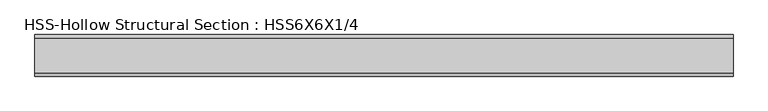
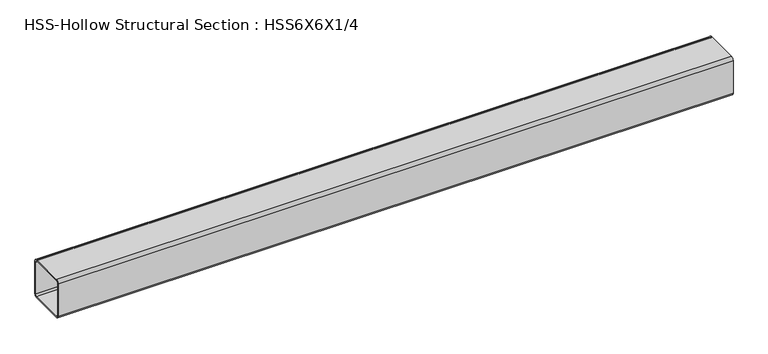
"""IFC4 building model written with IfcOpenShell, lengths in millimetres: beam geometry, HSS-Hollow Structural Section : HSS6X6X1/4."""

from ifc_helpers import new_model, si_unit, point, frame, frame_2d, origin, place, context, project, spatial, polyline, circle_curve, trimmed, segment, composite_curve, outline, extrude, source, transform, mapped, element, save


def hss_hollow_structural_section_hss6x6x1_4_a8101bfe(model_context):
    return source(origin(), model_context, "Body", "SweptSolid", [
        extrude(outline(composite_curve([segment(polyline([(76.2, 64.3636), (76.2, -64.3636)]), True, "CONTINUOUS"), segment(trimmed(circle_curve(frame_2d((64.3636, -64.3636)), 11.8364), [point((76.2, -64.3636))], [point((64.3636, -76.2))], False, "CARTESIAN"), True, "CONTINUOUS"), segment(polyline([(64.3636, -76.2), (-64.3636, -76.2)]), True, "CONTINUOUS"), segment(trimmed(circle_curve(frame_2d((-64.3636, -64.3636)), 11.8364), [point((-64.3636, -76.2))], [point((-76.2, -64.3636))], False, "CARTESIAN"), True, "CONTINUOUS"), segment(polyline([(-76.2, -64.3636), (-76.2, 64.3636)]), True, "CONTINUOUS"), segment(trimmed(circle_curve(frame_2d((-64.3636, 64.3636)), 11.8364), [point((-76.2, 64.3636))], [point((-64.3636, 76.2))], False, "CARTESIAN"), True, "CONTINUOUS"), segment(polyline([(-64.3636, 76.2), (64.3636, 76.2)]), True, "CONTINUOUS"), segment(trimmed(circle_curve(frame_2d((64.3636, 64.3636)), 11.8364), [point((64.3636, 76.2))], [point((76.2, 64.3636))], False, "CARTESIAN"), True, "CONTINUOUS")], self_intersect=False), holes=[composite_curve([segment(trimmed(circle_curve(frame_2d((-64.3636, 64.3636)), 5.9182), [point((-64.3636, 70.2818))], [point((-70.2818, 64.3636))], True, "CARTESIAN"), True, "CONTINUOUS"), segment(polyline([(-70.2818, 64.3636), (-70.2818, -64.3636)]), True, "CONTINUOUS"), segment(trimmed(circle_curve(frame_2d((-64.3636, -64.3636)), 5.9182), [point((-70.2818, -64.3636))], [point((-64.3636, -70.2818))], True, "CARTESIAN"), True, "CONTINUOUS"), segment(polyline([(-64.3636, -70.2818), (64.3636, -70.2818)]), True, "CONTINUOUS"), segment(trimmed(circle_curve(frame_2d((64.3636, -64.3636)), 5.9182), [point((64.3636, -70.2818))], [point((70.2818, -64.3636))], True, "CARTESIAN"), True, "CONTINUOUS"), segment(polyline([(70.2818, -64.3636), (70.2818, 64.3636)]), True, "CONTINUOUS"), segment(trimmed(circle_curve(frame_2d((64.3636, 64.3636)), 5.9182), [point((70.2818, 64.3636))], [point((64.3636, 70.2818))], True, "CARTESIAN"), True, "CONTINUOUS"), segment(polyline([(64.3636, 70.2818), (-64.3636, 70.2818)]), True, "CONTINUOUS")], self_intersect=False)]), frame((-1278.0540108, 0.0, 0.0), z_axis=(1.0, 0.0, 0.0), x_axis=(0.0, 1.0, 0.0)), (0.0, 0.0, 1.0), 2556.1080215),
    ])


if __name__ == "__main__":
    model = new_model("IFC4")
    model_context = context("Model", 3, world=origin())
    ifc_project = project(units=[si_unit("LENGTHUNIT", "METRE", prefix="MILLI")], contexts=[model_context])
    site = spatial("IfcSite", under=ifc_project)
    building = spatial("IfcBuilding", under=site)
    placement = place(None, origin())
    hss_hollow_structural_section_hss6x6x1_4_shape = hss_hollow_structural_section_hss6x6x1_4_a8101bfe(model_context)
    element("IfcBeam", 1, ObjectType="HSS-Hollow Structural Section : HSS6X6X1/4", at=placement, inside=building, context=model_context, shape_type="MappedRepresentation", body=[
        mapped(hss_hollow_structural_section_hss6x6x1_4_shape, transform((0.0, 0.0, 0.0), x_axis=(1.0, 0.0, 0.0), y_axis=(0.0, 1.0, 0.0), z_axis=(0.0, 0.0, 1.0))),
    ])
    save(model, "model.ifc")

# Revit data of these elements
# Type "HSS-Hollow Structural Section : HSS6X6X1/4"
#   Assembly Code = "B10"
#   Shape = "Square"
#   W = 19
#   Ht = 0' - 6"
#   Length [instance default] = 5' - 0"
#   b = 0' - 6"
#   kr = 0' - 0.466"
#   t = 0' - 0.233"
#   A = 0.0363889 SF
#   Structural Material [instance default] = Steel ASTM A500, Grade B, Rectangular and Square
# Element 1 (IfcBeam, "HSS-Hollow Structural Section : HSS6X6X1/4")
#   Materials on its faces: "Steel ASTM A500, Grade B, Rectangular and Square"
# Materials
#   "Steel ASTM A500, Grade B, Rectangular and Square": class "Metal", colour RGB 199 199 199, transparency 0, Description = "Carbon steel", Cost = 0
